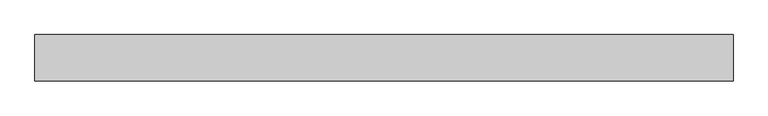
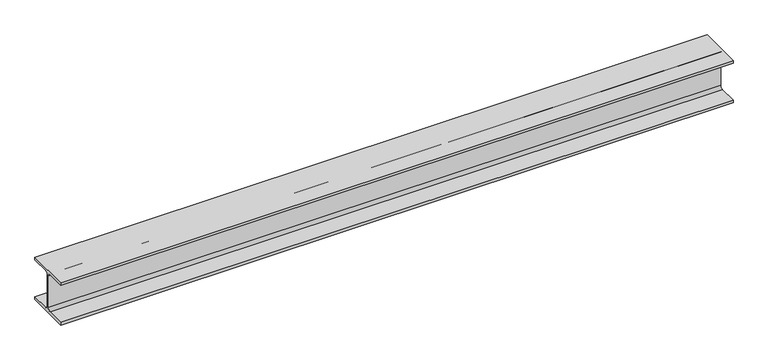
"""IFC4 building model written with IfcOpenShell, lengths in millimetres: beam geometry, 0912_Steel Framing_H-KSD3502 : H_SB_ASB_H-200x200x8x12."""

from ifc_helpers import new_model, si_unit, point, frame, frame_2d, origin, place, context, project, spatial, polyline, circle_curve, trimmed, segment, composite_curve, outline, extrude, source, transform, mapped, element, save


def beam_3227815b(model_context):
    return source(origin(), model_context, "Body", "SweptSolid", [
        extrude(outline(composite_curve([segment(polyline([(100.0, -88.0), (100.0, -100.0), (-100.0, -100.0), (-100.0, -88.0), (-17.0, -88.0)]), True, "CONTINUOUS"), segment(trimmed(circle_curve(frame_2d((-17.0, -75.0)), 13.0), [point((-17.0, -88.0))], [point((-4.0, -75.0))], True, "CARTESIAN"), True, "CONTINUOUS"), segment(polyline([(-4.0, -75.0), (-4.0, 75.0)]), True, "CONTINUOUS"), segment(trimmed(circle_curve(frame_2d((-17.0, 75.0)), 13.0), [point((-4.0, 75.0))], [point((-17.0, 88.0))], True, "CARTESIAN"), True, "CONTINUOUS"), segment(polyline([(-17.0, 88.0), (-100.0, 88.0), (-100.0, 100.0), (100.0, 100.0), (100.0, 88.0), (17.0, 88.0)]), True, "CONTINUOUS"), segment(trimmed(circle_curve(frame_2d((17.0, 75.0)), 13.0), [point((17.0, 88.0))], [point((4.0, 75.0))], True, "CARTESIAN"), True, "CONTINUOUS"), segment(polyline([(4.0, 75.0), (4.0, -75.0)]), True, "CONTINUOUS"), segment(trimmed(circle_curve(frame_2d((17.0, -75.0)), 13.0), [point((4.0, -75.0))], [point((17.0, -88.0))], True, "CARTESIAN"), True, "CONTINUOUS"), segment(polyline([(17.0, -88.0), (100.0, -88.0)]), True, "CONTINUOUS")], self_intersect=False)), frame((-1321.0203679, 0.0, 0.0), z_axis=(1.0, 0.0, 0.0), x_axis=(0.0, 1.0, 0.0)), (0.0, 0.0, 1.0), 3005.8055003),
    ])


if __name__ == "__main__":
    model = new_model("IFC4")
    model_context = context("Model", 3, world=origin())
    ifc_project = project(units=[si_unit("LENGTHUNIT", "METRE", prefix="MILLI")], contexts=[model_context])
    site = spatial("IfcSite", under=ifc_project)
    building = spatial("IfcBuilding", under=site)
    placement = place(None, origin())
    beam_shape = beam_3227815b(model_context)
    element("IfcBeam", 1, ObjectType="0912_Steel Framing_H-KSD3502 : H_SB_ASB_H-200x200x8x12", at=placement, inside=building, context=model_context, shape_type="MappedRepresentation", body=[
        mapped(beam_shape, transform((0.0, 0.0, 0.0), x_axis=(1.0, 0.0, 0.0), y_axis=(0.0, 1.0, 0.0), z_axis=(0.0, 0.0, 1.0))),
    ])
    save(model, "model.ifc")

# Revit data of these elements
# Type "0912_Steel Framing_H-KSD3502 : H_SB_ASB_H-200x200x8x12"
#   H_WM Code_1 = "S01AA002-00001 | Main Steel Structure Fabrication Work | Shelter/Building | Medium Steel - Standard (90KG/M>Weight≥30KG/M) | Material: (   )"
#   H_WM Code_2 = "S03AA028-00001 | Main Steel Structure Erection Work | Shelter/Building | Medium Steel (90KG/M>Weight≥30KG/M) | Material: (   )"
#   H_WM Code_3 = "S01AA010-00001 | Main Steel Structure Fabrication Work | Shelter/Building | Steel Painting/Coating | for Non-Fireproofed Steel Surface, Surface Preparation, Primer, Second & Final Coat | Material: (   )"
#   H_Q'ty Cal Type Tag = "SB-Q2"
#   Width = 20.0 cm
#   Web Thickness = 0.8 cm
#   Web Fillet = 1.3 cm
#   Warping Constant = 141000.0 cm⁶
#   W = 0
#   Torsional Moment of Inertia = 26.2485 cm⁴
#   Section Area = 63.53 cm²
#   Plastic Modulus weak axis = 244.0 cm³
#   Plastic Modulus strong axis = 525.0 cm³
#   Perimeter = 1.16 m²/m
#   Nominal Weight = 49.90 kgf/m
#   Moment of Inertia weak axis = 1600.00 cm⁴
#   Moment of Inertia strong axis = 4720.00 cm⁴
#   Height = 20.0 cm
#   Flange Thickness = 1.2 cm
#   Elastic Modulus weak axis = 160.0 cm³
#   Elastic Modulus strong axis = 472.0 cm³
#   Centroid Vertical = 10.0 cm
#   Centroid Horizontal = 10.0 cm
#   Ix = 47200000
#   Length [instance default] = 1.5240 m
#   Zx = 525000
#   b = 0.2000 m
#   h = 0.2000 m
#   r = 0.0130 m
#   s = 0.0080 m
#   t = 0.0120 m
#   A = 0.006353 m²
#   Structural Material [instance default] = Steel, 45-345
#   Assembly Code = ""
# Element 1 (IfcBeam, "0912_Steel Framing_H-KSD3502 : H_SB_ASB_H-200x200x8x12")
#   Structural Material = none
# Materials
#   "Steel, 45-345": class "Metal", colour RGB 189 187 185, transparency 0, Description = "Steel 345 MPa", Cost = 0
